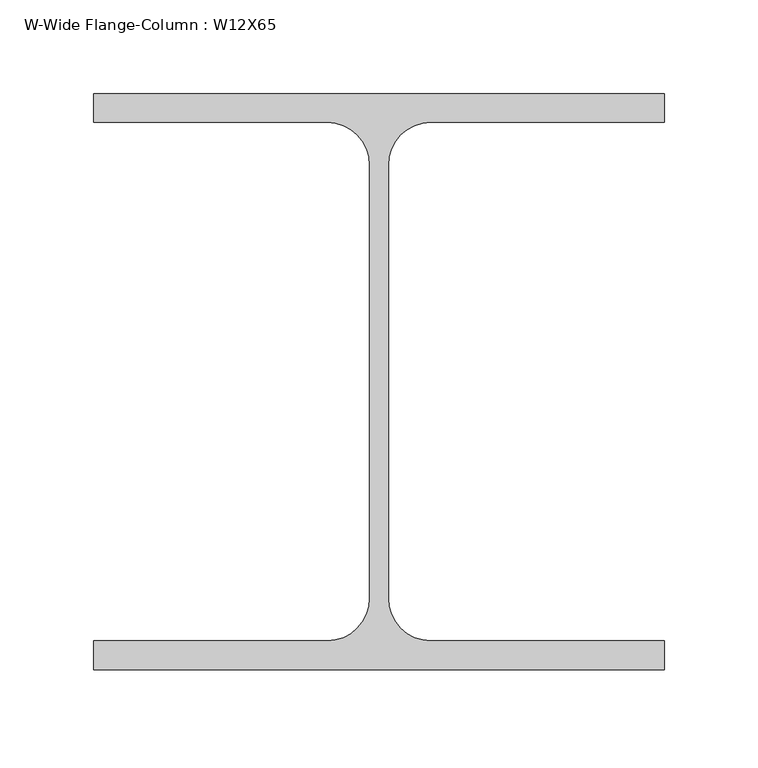
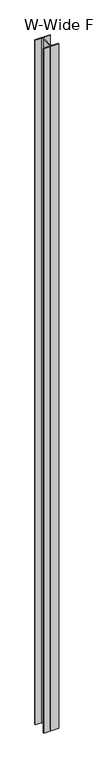
"""IFC4 building model written with IfcOpenShell, lengths in millimetres: column geometry, W-Wide Flange-Column : W12X65."""

from ifc_helpers import new_model, si_unit, point, frame, frame_2d, origin, place, context, project, spatial, polyline, circle_curve, trimmed, segment, composite_curve, outline, extrude, source, transform, mapped, element, save


def w_wide_flange_column_w12x65_b7a4a025(model_context):
    return source(origin(), model_context, "Body", "SweptSolid", [
        extrude(outline(composite_curve([segment(polyline([(152.4, 153.67), (152.4, 138.303), (27.686, 138.303)]), True, "CONTINUOUS"), segment(trimmed(circle_curve(frame_2d((27.686, 115.57)), 22.733), [point((27.686, 138.303))], [point((4.953, 115.57))], True, "CARTESIAN"), True, "CONTINUOUS"), segment(polyline([(4.953, 115.57), (4.953, -115.57)]), True, "CONTINUOUS"), segment(trimmed(circle_curve(frame_2d((27.686, -115.57)), 22.733), [point((4.953, -115.57))], [point((27.686, -138.303))], True, "CARTESIAN"), True, "CONTINUOUS"), segment(polyline([(27.686, -138.303), (152.4, -138.303), (152.4, -153.67), (-152.4, -153.67), (-152.4, -138.303), (-27.686, -138.303)]), True, "CONTINUOUS"), segment(trimmed(circle_curve(frame_2d((-27.686, -115.57)), 22.733), [point((-27.686, -138.303))], [point((-4.953, -115.57))], True, "CARTESIAN"), True, "CONTINUOUS"), segment(polyline([(-4.953, -115.57), (-4.953, 115.57)]), True, "CONTINUOUS"), segment(trimmed(circle_curve(frame_2d((-27.686, 115.57)), 22.733), [point((-4.953, 115.57))], [point((-27.686, 138.303))], True, "CARTESIAN"), True, "CONTINUOUS"), segment(polyline([(-27.686, 138.303), (-152.4, 138.303), (-152.4, 153.67), (152.4, 153.67)]), True, "CONTINUOUS")], self_intersect=False)), frame((0.0, 0.0, 8756.65), z_axis=(0.0, 0.0, 1.0), x_axis=(1.0, 0.0, 0.0)), (0.0, 0.0, 1.0), 14560.55),
    ])


if __name__ == "__main__":
    model = new_model("IFC4")
    model_context = context("Model", 3, world=origin())
    ifc_project = project(units=[si_unit("LENGTHUNIT", "METRE", prefix="MILLI")], contexts=[model_context])
    site = spatial("IfcSite", under=ifc_project)
    building = spatial("IfcBuilding", under=site)
    placement = place(None, origin())
    w_wide_flange_column_w12x65_shape = w_wide_flange_column_w12x65_b7a4a025(model_context)
    element("IfcColumn", 1, ObjectType="W-Wide Flange-Column : W12X65", at=placement, inside=building, context=model_context, shape_type="MappedRepresentation", body=[
        mapped(w_wide_flange_column_w12x65_shape, transform((0.0, 0.0, 0.0), x_axis=(1.0, 0.0, 0.0), y_axis=(0.0, 1.0, 0.0), z_axis=(0.0, 0.0, 1.0))),
    ])
    save(model, "model.ifc")

# Revit data of these elements
# Type "W-Wide Flange-Column : W12X65"
#   Assembly Code = "B10"
#   W = 65
#   bf = 1' - 0"
#   d = 1' - 0.1"
#   k = 0' - 1 1/2"
#   kr = 0' - 0.895"
#   tf = 0' - 0.605"
#   tw = 0' - 0.39"
#   A = 0.132639 SF
#   Structural Material [instance default] = Steel ASTM A992
# Element 1 (IfcColumn, "W-Wide Flange-Column : W12X65")
#   Materials on its faces: "Steel ASTM A992"
# Materials
#   "Steel ASTM A992": class "Metal", colour RGB 199 199 199, transparency 0, Description = "Structural steel 50ksi", Cost = 0
